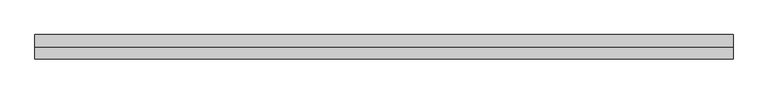
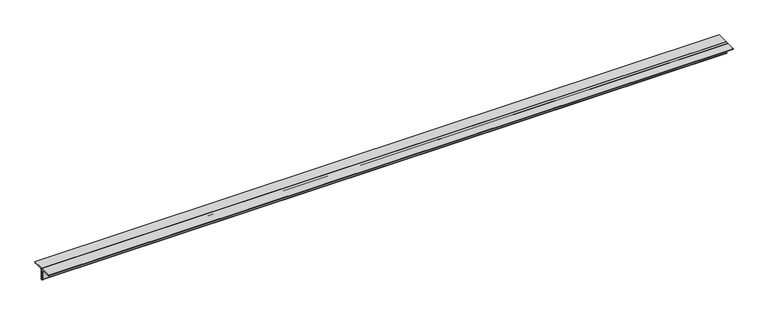
"""IFC4 building model written with IfcOpenShell, lengths in millimetres: member geometry, 0123_Steel Framing_2Ls-KSD3502 : H_SB_AR_S04_2Ls-130x130x12_VBR2."""

from ifc_helpers import new_model, si_unit, point, frame, frame_2d, origin, place, context, project, spatial, polyline, circle_curve, trimmed, segment, composite_curve, outline, extrude, source, transform, mapped, element, save


def member_9903f92b(model_context):
    return source(origin(), model_context, "Body", "SweptSolid", [
        extrude(outline(composite_curve([segment(polyline([(0.0, 36.4), (130.0, 36.4)]), True, "CONTINUOUS"), segment(trimmed(circle_curve(frame_2d((118.0, 36.4)), 12.0), [point((130.0, 36.4))], [point((118.0, 24.4))], False, "CARTESIAN"), True, "CONTINUOUS"), segment(polyline([(118.0, 24.4), (24.0, 24.4)]), True, "CONTINUOUS"), segment(trimmed(circle_curve(frame_2d((24.0, 12.4)), 12.0), [point((24.0, 24.4))], [point((12.0, 12.4))], True, "CARTESIAN"), True, "CONTINUOUS"), segment(polyline([(12.0, 12.4), (12.0, -81.6)]), True, "CONTINUOUS"), segment(trimmed(circle_curve(frame_2d((0.0, -81.6)), 12.0), [point((12.0, -81.6))], [point((0.0, -93.6))], False, "CARTESIAN"), True, "CONTINUOUS"), segment(polyline([(0.0, -93.6), (0.0, 36.4)]), True, "CONTINUOUS")], self_intersect=False)), frame((-3854.8431433, 0.0, 0.0), z_axis=(1.0, 0.0, 0.0), x_axis=(0.0, 1.0, 0.0)), (0.0, 0.0, 1.0), 7389.5605416),
        extrude(outline(composite_curve([segment(polyline([(0.0, 36.4), (0.0, -93.6)]), True, "CONTINUOUS"), segment(trimmed(circle_curve(frame_2d((0.0, -81.6)), 12.0), [point((0.0, -93.6))], [point((-12.0, -81.6))], False, "CARTESIAN"), True, "CONTINUOUS"), segment(polyline([(-12.0, -81.6), (-12.0, 12.4)]), True, "CONTINUOUS"), segment(trimmed(circle_curve(frame_2d((-24.0, 12.4)), 12.0), [point((-12.0, 12.4))], [point((-24.0, 24.4))], True, "CARTESIAN"), True, "CONTINUOUS"), segment(polyline([(-24.0, 24.4), (-118.0, 24.4)]), True, "CONTINUOUS"), segment(trimmed(circle_curve(frame_2d((-118.0, 36.4)), 12.0), [point((-118.0, 24.4))], [point((-130.0, 36.4))], False, "CARTESIAN"), True, "CONTINUOUS"), segment(polyline([(-130.0, 36.4), (0.0, 36.4)]), True, "CONTINUOUS")], self_intersect=False)), frame((-3854.8431433, 0.0, 0.0), z_axis=(1.0, 0.0, 0.0), x_axis=(0.0, 1.0, 0.0)), (0.0, 0.0, 1.0), 7389.5605416),
    ])


if __name__ == "__main__":
    model = new_model("IFC4")
    model_context = context("Model", 3, world=origin())
    ifc_project = project(units=[si_unit("LENGTHUNIT", "METRE", prefix="MILLI")], contexts=[model_context])
    site = spatial("IfcSite", under=ifc_project)
    building = spatial("IfcBuilding", under=site)
    placement = place(None, origin())
    member_shape = member_9903f92b(model_context)
    element("IfcMember", 1, ObjectType="0123_Steel Framing_2Ls-KSD3502 : H_SB_AR_S04_2Ls-130x130x12_VBR2", at=placement, inside=building, context=model_context, shape_type="MappedRepresentation", body=[
        mapped(member_shape, transform((0.0, 0.0, 0.0), x_axis=(1.0, 0.0, 0.0), y_axis=(0.0, 1.0, 0.0), z_axis=(0.0, 0.0, 1.0))),
    ])
    save(model, "model.ifc")

# Revit data of these elements
# Type "0123_Steel Framing_2Ls-KSD3502 : H_SB_AR_S04_2Ls-130x130x12_VBR2"
#   Assembly Code = "B10"
#   Legs = "SLBB"
#   W = 8.97
#   Perimeter = 1.04 m²/m
#   Nominal Weight = 46.80 kgf/m
#   Length [instance default] = 1000 mm
#   Space = 0 mm
#   b = 130 mm
#   d = 130 mm
#   t = 12 mm
#   y = 36.4 mm
#   A = 0.005952 m²
#   Structural Material [instance default] = Steel ASTM A36
# Element 1 (IfcMember, "0123_Steel Framing_2Ls-KSD3502 : H_SB_AR_S04_2Ls-130x130x12_VBR2")
#   Structural Material = Steel, 45-345
#   Materials on its faces: "Steel, 45-345"
# Materials
#   "Steel ASTM A36": class "Metal", colour RGB 199 199 199, transparency 0, Description = "Structural steel, ASTM A36 Grade B, mill finish", Cost = 0
#   "Steel, 45-345": class "Metal", colour RGB 189 187 185, transparency 0, Description = "Steel 345 MPa", Cost = 0
